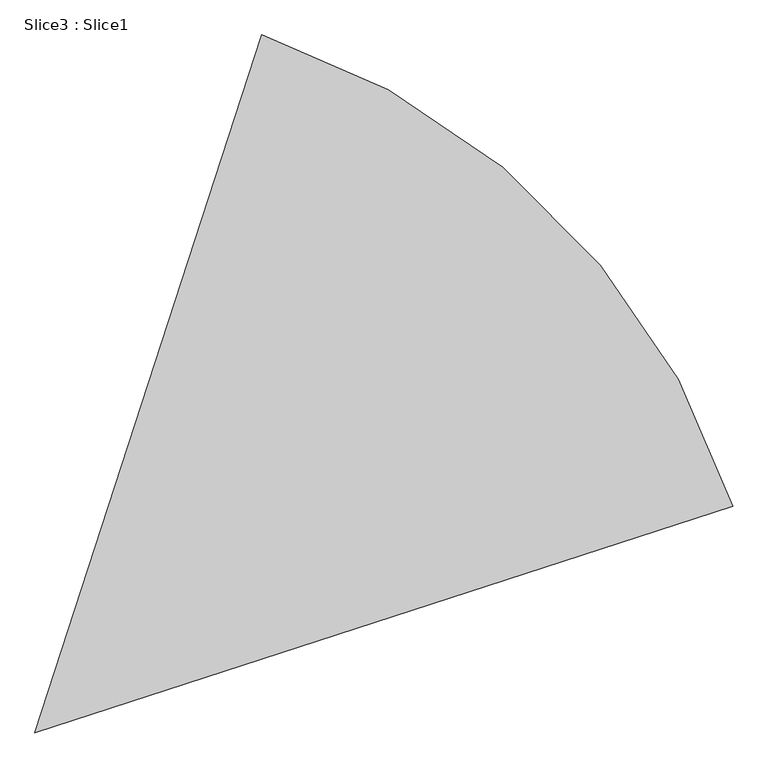
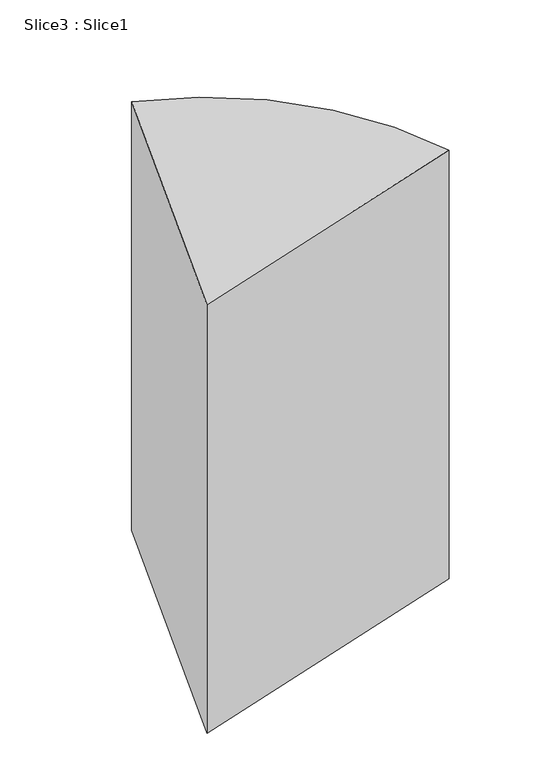
"""IFC4 building model written with IfcOpenShell, lengths in millimetres: proxy geometry, Slice3 : Slice1."""

from ifc_helpers import new_model, si_unit, point, origin, origin_with_axes, origin_2d, place, context, project, spatial, polyline, circle_curve, trimmed, segment, composite_curve, outline, extrude, source, transform, mapped, element, save


def slice3_slice1_d857eb85(model_context):
    return source(origin(), model_context, "Body", "SweptSolid", [
        extrude(outline(composite_curve([segment(trimmed(circle_curve(origin_2d(), 1100.0), [point((339.9186938, 1046.1621679))], [point((1046.1621679, 339.9186938))], False, "CARTESIAN"), True, "CONTINUOUS"), segment(polyline([(1046.1621679, 339.9186938), (0.0, 0.0), (339.9186938, 1046.1621679)]), True, "CONTINUOUS")], self_intersect=False)), origin_with_axes(), (0.0, 0.0, 1.0), 1589.6460515),
    ])


if __name__ == "__main__":
    model = new_model("IFC4")
    model_context = context("Model", 3, world=origin())
    ifc_project = project(units=[si_unit("LENGTHUNIT", "METRE", prefix="MILLI")], contexts=[model_context])
    site = spatial("IfcSite", under=ifc_project)
    building = spatial("IfcBuilding", under=site)
    placement = place(None, origin())
    slice3_slice1_shape = slice3_slice1_d857eb85(model_context)
    element("IfcBuildingElementProxy", 1, Name="Slice3 : Slice1", ObjectType="Slice3 : Slice1", at=placement, inside=building, context=model_context, shape_type="MappedRepresentation", body=[
        mapped(slice3_slice1_shape, transform((0.0, 0.0, 0.0), x_axis=(1.0, 0.0, 0.0), y_axis=(0.0, 1.0, 0.0), z_axis=(0.0, 0.0, 1.0))),
    ])
    save(model, "model.ifc")
